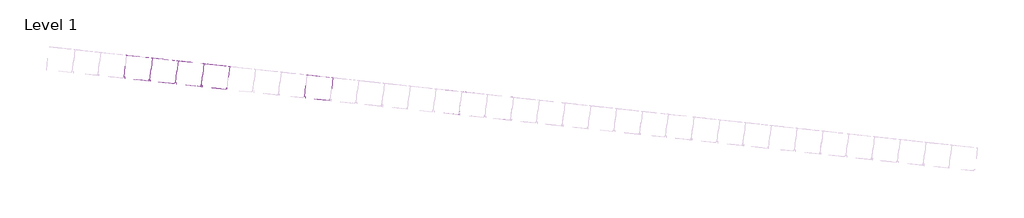
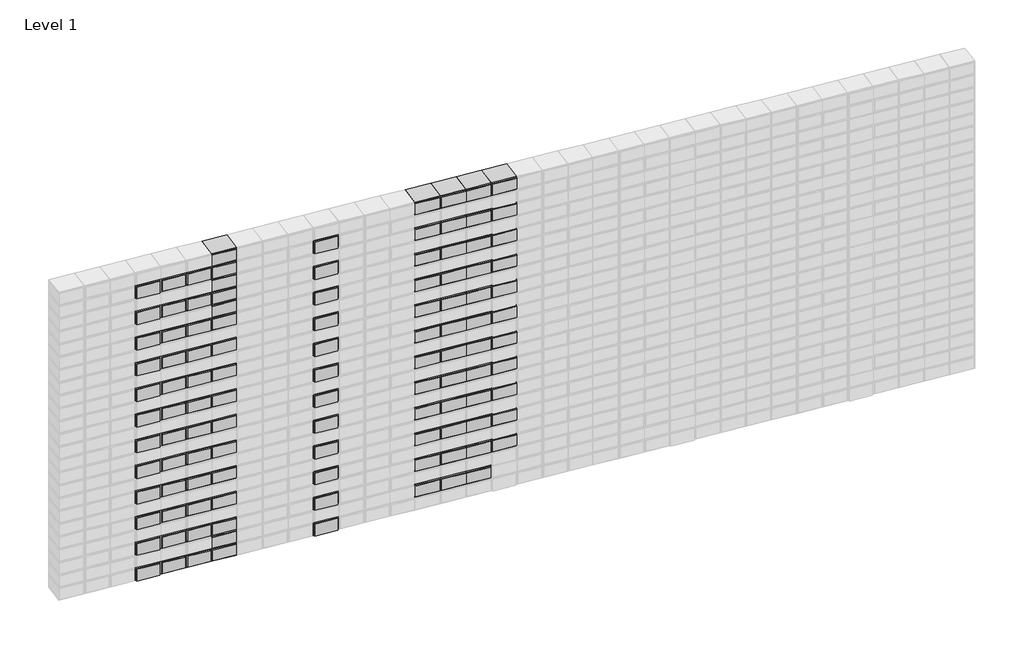
# One storey, part 13 of 18: 111 proxies.
"""IFC4 building model written with IfcOpenShell, lengths in millimetres."""

import ifcopenshell
import ifcopenshell.guid

model = None  # the IFC model being written
_history = None  # IfcOwnerHistory: only IFC2X3 demands one
_inside = {}  # id of a spatial element -> (the spatial element, [elements in it])
_under = {}  # id of a project, library or spatial element -> (it, [spatial elements below it])
_declared = {}  # id of a project -> (the project, [libraries it declares])
_typed = {}  # id of a type object -> (the type object, [elements of that type])
_made_of = {}  # id of a material, layer set ... -> (it, [elements and type objects made of it])


def new_model(schema):
    """Start an empty IFC model of exactly this schema.

    Asked for "IFC4X3", IfcOpenShell would pick the latest addendum, in which some entities
    have other attributes; the version numbers below select the first issue.
    IFC2X3 requires an IfcOwnerHistory on every rooted entity: one is made here for all.
    """
    global model, _history
    if schema == "IFC4X3":
        model = ifcopenshell.file(schema_version=(4, 3, 0, 0))
    else:
        model = ifcopenshell.file(schema=schema)
    _inside.clear()
    _under.clear()
    _declared.clear()
    _typed.clear()
    _made_of.clear()
    _history = None
    if model.schema == "IFC2X3":
        org = make("IfcOrganization", Name="unknown")
        user = make(
            "IfcPersonAndOrganization",
            ThePerson=make("IfcPerson", FamilyName="unknown"),
            TheOrganization=org,
        )
        app = make(
            "IfcApplication",
            ApplicationDeveloper=org,
            Version="unknown",
            ApplicationFullName="unknown",
            ApplicationIdentifier="unknown",
        )
        _history = make(
            "IfcOwnerHistory",
            OwningUser=user,
            OwningApplication=app,
            ChangeAction="ADDED",
            CreationDate=0,
        )
    return model


def make(cls, **values):
    """One entity of the class cls with the attributes given. An attribute that is None is left unset."""
    return model.create_entity(
        cls, **{name: value for name, value in values.items() if value is not None}
    )


def rooted(cls, **values):
    """An entity with a GlobalId (a new one), such as an element, a storey or a relation."""
    return make(cls, GlobalId=ifcopenshell.guid.new(), OwnerHistory=_history, **values)


def si_unit(unit_type, name, prefix=None):
    """IfcSIUnit, for example si_unit("LENGTHUNIT", "METRE", prefix="MILLI")."""
    return make("IfcSIUnit", UnitType=unit_type, Prefix=prefix, Name=name)


def assignment(units):
    """IfcUnitAssignment: the units of a project."""
    return None if units is None else make("IfcUnitAssignment", Units=units)


def point(xyz):
    """IfcCartesianPoint."""
    return None if xyz is None else make("IfcCartesianPoint", Coordinates=xyz)


def direction(xyz):
    """IfcDirection."""
    return None if xyz is None else make("IfcDirection", DirectionRatios=xyz)


def frame(location, z_axis=None, x_axis=None):
    """IfcAxis2Placement3D, a coordinate frame: its origin and axes. An axis left out is left unset."""
    return make(
        "IfcAxis2Placement3D",
        Location=point(location),
        Axis=direction(z_axis),
        RefDirection=direction(x_axis),
    )


def origin():
    """The frame at (0, 0, 0) with its axes left unset."""
    return frame((0.0, 0.0, 0.0))


def origin_with_axes():
    """The frame at (0, 0, 0) with the z axis (0, 0, 1) and the x axis (1, 0, 0) written out."""
    return frame((0.0, 0.0, 0.0), z_axis=(0.0, 0.0, 1.0), x_axis=(1.0, 0.0, 0.0))


def place(relative_to, where):
    """IfcLocalPlacement: puts the frame where relative to a parent placement (None: the world)."""
    return make(
        "IfcLocalPlacement", PlacementRelTo=relative_to, RelativePlacement=where
    )


def context(
    kind, dimensions, precision=None, world=None, true_north=None, identifier=None
):
    """IfcGeometricRepresentationContext, for example the 3D "Model" context."""
    return make(
        "IfcGeometricRepresentationContext",
        ContextIdentifier=identifier,
        ContextType=kind,
        CoordinateSpaceDimension=dimensions,
        Precision=precision,
        WorldCoordinateSystem=world,
        TrueNorth=true_north,
    )


def project(units=None, contexts=None):
    """IfcProject with its units and contexts."""
    return rooted(
        "IfcProject",
        Name="project",
        RepresentationContexts=contexts,
        UnitsInContext=assignment(units),
    )


def spatial(cls, under=None, at=None, **own):
    """A site, building, storey or space (cls), placed at a placement, below another one or the project."""
    s = rooted(cls, ObjectPlacement=at, **own)
    if under is not None:
        _under.setdefault(under.id(), (under, []))[1].append(s)
    return s


def polyline(points):
    """IfcPolyline through the points."""
    return make("IfcPolyline", Points=[point(p) for p in points])


def outline(outer, holes=None, kind="AREA"):
    """IfcArbitraryClosedProfileDef: a profile drawn as a closed curve; with holes, ...WithVoids."""
    if holes is None:
        return make("IfcArbitraryClosedProfileDef", ProfileType=kind, OuterCurve=outer)
    return make(
        "IfcArbitraryProfileDefWithVoids",
        ProfileType=kind,
        OuterCurve=outer,
        InnerCurves=holes,
    )


def extrude(swept, where, along, depth):
    """IfcExtrudedAreaSolid: the profile swept, set in the frame where, extruded along a direction by depth."""
    return make(
        "IfcExtrudedAreaSolid",
        SweptArea=swept,
        Position=where,
        ExtrudedDirection=direction(along),
        Depth=depth,
    )


def shape(context_of_items, identifier, shape_type, items):
    """IfcShapeRepresentation: the items that make up one representation, for example the "Body"."""
    return make(
        "IfcShapeRepresentation",
        ContextOfItems=context_of_items,
        RepresentationIdentifier=identifier,
        RepresentationType=shape_type,
        Items=items,
    )


def source(mapping_origin, context_of_items, identifier, shape_type, items):
    """IfcRepresentationMap: a shape defined once, which mapped items show again and again."""
    return make(
        "IfcRepresentationMap",
        MappingOrigin=mapping_origin,
        MappedRepresentation=shape(context_of_items, identifier, shape_type, items),
    )


def transform(
    local_origin,
    x_axis=None,
    y_axis=None,
    z_axis=None,
    scale=None,
    scale2=None,
    scale3=None,
    uniform=True,
):
    """IfcCartesianTransformationOperator3D, or its non-uniform kind. x_axis, y_axis, z_axis: its Axis1, 2, 3."""
    if uniform:
        return make(
            "IfcCartesianTransformationOperator3D",
            Axis1=direction(x_axis),
            Axis2=direction(y_axis),
            LocalOrigin=point(local_origin),
            Scale=scale,
            Axis3=direction(z_axis),
        )
    return make(
        "IfcCartesianTransformationOperator3DnonUniform",
        Axis1=direction(x_axis),
        Axis2=direction(y_axis),
        LocalOrigin=point(local_origin),
        Scale=scale,
        Axis3=direction(z_axis),
        Scale2=scale2,
        Scale3=scale3,
    )


def mapped(mapping_source, mapping_target):
    """IfcMappedItem: shows the shape of a source again, moved by a transform."""
    return make(
        "IfcMappedItem", MappingSource=mapping_source, MappingTarget=mapping_target
    )


def made_of(thing, what):
    """Note that an element or type object is made of a material, layer set ...; save() writes the relation."""
    if what is not None:
        _made_of.setdefault(what.id(), (what, []))[1].append(thing)
    return thing


def element(
    cls,
    number,
    at=None,
    inside=None,
    cuts=None,
    type_object=None,
    material=None,
    context=None,
    identifier="Body",
    shape_type=None,
    held_by="IfcProductDefinitionShape",
    body=None,
    shapes=None,
    **own,
):
    """One element of the class cls, such as IfcWall. Its Tag is "e" and its number.

    at: its placement. inside: the storey or other place that contains it. cuts: it is an
    opening in that element (IfcRelVoidsElement). A single representation is given by context,
    identifier, shape_type and body (its items); several are given by shapes. held_by: the class
    of the entity that holds the representations. save() writes the other relations.
    """
    e = rooted(cls, Tag="e%d" % number, ObjectPlacement=at, **own)
    if body is not None:
        shapes = [shape(context, identifier, shape_type, body)]
    if shapes is not None:
        e.Representation = make(held_by, Representations=shapes)
    if inside is not None:
        _inside.setdefault(inside.id(), (inside, []))[1].append(e)
    if cuts is not None:
        rooted(
            "IfcRelVoidsElement", RelatingBuildingElement=cuts, RelatedOpeningElement=e
        )
    if type_object is not None:
        _typed.setdefault(type_object.id(), (type_object, []))[1].append(e)
    return made_of(e, material)


def aggregate(whole, parts):
    """IfcRelAggregates: a whole, such as a stair, and the parts it consists of."""
    return rooted("IfcRelAggregates", RelatingObject=whole, RelatedObjects=parts)


def save(model, path):
    """Write the relations noted so far, then the file.

    IfcRelAggregates (storeys below a building ...), IfcRelContainedInSpatialStructure (elements
    in a storey), IfcRelDefinesByType, IfcRelAssociatesMaterial and IfcRelDeclares: one each for
    every whole, place, type object, material and project.
    """
    for whole, parts in _under.values():
        aggregate(whole, parts)
    for where, things in _inside.values():
        rooted(
            "IfcRelContainedInSpatialStructure",
            RelatedElements=things,
            RelatingStructure=where,
        )
    for kind, things in _typed.values():
        rooted("IfcRelDefinesByType", RelatedObjects=things, RelatingType=kind)
    for what, things in _made_of.values():
        rooted("IfcRelAssociatesMaterial", RelatedObjects=things, RelatingMaterial=what)
    for by, libraries in _declared.values():
        rooted("IfcRelDeclares", RelatingContext=by, RelatedDefinitions=libraries)
    model.write(path)


def geel_a5fc7152(model_context):
    return source(origin(), model_context, "Body", "SweptSolid", [
        extrude(outline(polyline([(131.1871262, 51.8695461), (24.8461542, 24.0369432), (23.5801491, 28.8740117), (125.0840527, 55.4406095), (111.9430518, 105.6488784), (10.4391482, 79.0822806), (9.1731432, 83.919349), (115.5141152, 111.7519519), (131.1871262, 51.8695461)])), origin_with_axes(), (0.0, 0.0, 1.0), 95.0),
        extrude(outline(polyline([(111.9430518, 105.6488784), (125.0840527, 55.4406095), (23.5801491, 28.8740117), (10.4391482, 79.0822806), (111.9430518, 105.6488784)])), origin_with_axes(), (0.0, 0.0, 1.0), 100.0),
    ])


def geel_ff5a4212(model_context):
    return source(origin(), model_context, "Body", "SweptSolid", [
        extrude(outline(polyline([(24.8461542, 24.0369432), (9.1731432, 83.919349), (115.5141152, 111.7519519), (116.7801202, 106.9148835), (15.2762167, 80.3482856), (28.4172176, 30.1400167), (129.9211211, 56.7066146), (131.1871262, 51.8695461), (24.8461542, 24.0369432)])), origin_with_axes(), (0.0, 0.0, 1.0), 95.0),
        extrude(outline(polyline([(116.7801202, 106.9148835), (129.9211211, 56.7066146), (28.4172176, 30.1400167), (15.2762167, 80.3482856), (116.7801202, 106.9148835)])), origin_with_axes(), (0.0, 0.0, 1.0), 100.0),
    ])


def rood_14a66368(model_context):
    return source(origin(), model_context, "Body", "SweptSolid", [
        extrude(outline(polyline([(24.8461542, 24.0369432), (9.1731432, 83.919349), (115.5141152, 111.7519519), (131.1871262, 51.8695461), (24.8461542, 24.0369432)]), holes=[polyline([(125.0840527, 55.4406095), (111.9430518, 105.6488784), (15.2762167, 80.3482856), (28.4172176, 30.1400167), (125.0840527, 55.4406095)])]), origin_with_axes(), (0.0, 0.0, 1.0), 95.0),
        extrude(outline(polyline([(111.9430518, 105.6488784), (125.0840527, 55.4406095), (28.4172176, 30.1400167), (15.2762167, 80.3482856), (111.9430518, 105.6488784)])), origin_with_axes(), (0.0, 0.0, 1.0), 100.0),
    ])


def rood_2ddd8018(model_context):
    return source(origin(), model_context, "Body", "SweptSolid", [
        extrude(outline(polyline([(24.8461542, 24.0369432), (9.1731432, 83.919349), (115.5141152, 111.7519519), (131.1871262, 51.8695461), (126.3500577, 50.6035411), (111.9430518, 105.6488784), (15.2762167, 80.3482856), (29.6832226, 25.3029482), (24.8461542, 24.0369432)])), origin_with_axes(), (0.0, 0.0, 1.0), 95.0),
        extrude(outline(polyline([(111.9430518, 105.6488784), (126.3500577, 50.6035411), (29.6832226, 25.3029482), (15.2762167, 80.3482856), (111.9430518, 105.6488784)])), origin_with_axes(), (0.0, 0.0, 1.0), 100.0),
    ])


model = new_model("IFC4")

# Units and contexts
model_context = context("Model", 3, world=origin())
ifc_project = project(units=[si_unit("LENGTHUNIT", "METRE", prefix="MILLI")], contexts=[model_context])

# Site, building, storey
site = spatial("IfcSite", under=ifc_project)
building = spatial("IfcBuilding", under=site)
storey = spatial("IfcBuildingStorey", under=building, Name="Level 1", Elevation=0.0)

# Proxies
placement = place(None, origin())
geel_shape = geel_a5fc7152(model_context)
element("IfcBuildingElementProxy", 1, Name="Geel", ObjectType="Geel", at=placement, inside=storey, context=model_context, shape_type="MappedRepresentation", body=[
    mapped(geel_shape, transform((10406.9656935, -4442.8724558, 2168.7358475), x_axis=(0.9617275503729374, -0.1047347566147725, -0.25320100633787673), y_axis=(0.25171277368869216, -0.02741220845642974, 0.9674136914420255), z_axis=(-0.10826263628609081, -0.9941223272738551, 0.0))),
])
element("IfcBuildingElementProxy", 2, Name="Geel", ObjectType="Geel", at=placement, inside=storey, context=model_context, shape_type="MappedRepresentation", body=[
    mapped(geel_shape, transform((10406.9656935, -4442.8724558, 2292.5348104), x_axis=(0.9617275503729374, -0.1047347566147725, -0.25320100633787673), y_axis=(0.25171277368869216, -0.02741220845642974, 0.9674136914420255), z_axis=(-0.10826263628609081, -0.9941223272738551, 0.0))),
])
element("IfcBuildingElementProxy", 3, Name="Geel", ObjectType="Geel", at=placement, inside=storey, context=model_context, shape_type="MappedRepresentation", body=[
    mapped(geel_shape, transform((10406.9656935, -4442.8724558, 2416.3337732), x_axis=(0.9617275503729384, -0.1047347566147726, -0.25320100633787307), y_axis=(0.25171277368868855, -0.02741220845642934, 0.9674136914420265), z_axis=(-0.10826263628609081, -0.994122327273855, 0.0))),
])
element("IfcBuildingElementProxy", 4, Name="Geel", ObjectType="Geel", at=placement, inside=storey, context=model_context, shape_type="MappedRepresentation", body=[
    mapped(geel_shape, transform((10406.9656935, -4442.8724558, 2540.132736), x_axis=(0.9617275503729374, -0.1047347566147725, -0.25320100633787673), y_axis=(0.25171277368869216, -0.02741220845642974, 0.9674136914420255), z_axis=(-0.10826263628609081, -0.9941223272738551, 0.0))),
])
element("IfcBuildingElementProxy", 5, Name="Geel", ObjectType="Geel", at=placement, inside=storey, context=model_context, shape_type="MappedRepresentation", body=[
    mapped(geel_shape, transform((10406.9656935, -4442.8724558, 2663.9316989), x_axis=(0.9617275503729374, -0.1047347566147725, -0.25320100633787673), y_axis=(0.25171277368869216, -0.02741220845642974, 0.9674136914420255), z_axis=(-0.10826263628609081, -0.9941223272738551, 0.0))),
])
element("IfcBuildingElementProxy", 6, Name="Geel", ObjectType="Geel", at=placement, inside=storey, context=model_context, shape_type="MappedRepresentation", body=[
    mapped(geel_shape, transform((10406.9656935, -4442.8724558, 2787.7306617), x_axis=(0.9617275503729374, -0.1047347566147725, -0.25320100633787673), y_axis=(0.25171277368869216, -0.02741220845642974, 0.9674136914420255), z_axis=(-0.10826263628609081, -0.9941223272738551, 0.0))),
])
element("IfcBuildingElementProxy", 7, Name="Geel", ObjectType="Geel", at=placement, inside=storey, context=model_context, shape_type="MappedRepresentation", body=[
    mapped(geel_shape, transform((10406.9656935, -4442.8724558, 2911.5296245), x_axis=(0.9617275503729374, -0.1047347566147725, -0.25320100633787673), y_axis=(0.25171277368869216, -0.02741220845642974, 0.9674136914420255), z_axis=(-0.10826263628609081, -0.9941223272738551, 0.0))),
])
element("IfcBuildingElementProxy", 8, Name="Geel", ObjectType="Geel", at=placement, inside=storey, context=model_context, shape_type="MappedRepresentation", body=[
    mapped(geel_shape, transform((10406.9656935, -4442.8724558, 3035.3285874), x_axis=(0.9617275503729374, -0.1047347566147725, -0.25320100633787673), y_axis=(0.25171277368869216, -0.02741220845642974, 0.9674136914420255), z_axis=(-0.10826263628609081, -0.9941223272738551, 0.0))),
])
element("IfcBuildingElementProxy", 9, Name="Geel", ObjectType="Geel", at=placement, inside=storey, context=model_context, shape_type="MappedRepresentation", body=[
    mapped(geel_shape, transform((10406.9656935, -4442.8724558, 3159.1275502), x_axis=(0.9617275503729374, -0.1047347566147725, -0.25320100633787673), y_axis=(0.25171277368869216, -0.02741220845642974, 0.9674136914420255), z_axis=(-0.10826263628609081, -0.9941223272738551, 0.0))),
])
element("IfcBuildingElementProxy", 10, Name="Geel", ObjectType="Geel", at=placement, inside=storey, context=model_context, shape_type="MappedRepresentation", body=[
    mapped(geel_shape, transform((10406.9656935, -4442.8724558, 3282.926513), x_axis=(0.9617275503729374, -0.1047347566147725, -0.25320100633787673), y_axis=(0.25171277368869216, -0.02741220845642974, 0.9674136914420255), z_axis=(-0.10826263628609081, -0.9941223272738551, 0.0))),
])
element("IfcBuildingElementProxy", 11, Name="Geel", ObjectType="Geel", at=placement, inside=storey, context=model_context, shape_type="MappedRepresentation", body=[
    mapped(geel_shape, transform((10406.9656935, -4442.8724558, 3406.7254759), x_axis=(0.9617275503729374, -0.1047347566147725, -0.25320100633787673), y_axis=(0.25171277368869216, -0.02741220845642974, 0.9674136914420255), z_axis=(-0.10826263628609081, -0.9941223272738551, 0.0))),
])
element("IfcBuildingElementProxy", 12, Name="Geel", ObjectType="Geel", at=placement, inside=storey, context=model_context, shape_type="MappedRepresentation", body=[
    mapped(geel_shape, transform((10406.9656935, -4442.8724558, 2044.9368847), x_axis=(0.9617275503729384, -0.1047347566147726, -0.25320100633787307), y_axis=(0.25171277368868855, -0.02741220845642934, 0.9674136914420265), z_axis=(-0.10826263628609081, -0.994122327273855, 0.0))),
])
element("IfcBuildingElementProxy", 13, Name="Geel", ObjectType="Geel", at=placement, inside=storey, context=model_context, shape_type="MappedRepresentation", body=[
    mapped(geel_shape, transform((10625.5194219, -4466.6735537, 2168.7358475), x_axis=(0.9617275503729374, -0.1047347566147725, -0.25320100633787673), y_axis=(0.25171277368869216, -0.02741220845642974, 0.9674136914420255), z_axis=(-0.10826263628609081, -0.9941223272738551, 0.0))),
])
element("IfcBuildingElementProxy", 14, Name="Geel", ObjectType="Geel", at=placement, inside=storey, context=model_context, shape_type="MappedRepresentation", body=[
    mapped(geel_shape, transform((10625.5194219, -4466.6735537, 2292.5348104), x_axis=(0.9617275503729374, -0.1047347566147725, -0.25320100633787673), y_axis=(0.25171277368869216, -0.02741220845642974, 0.9674136914420255), z_axis=(-0.10826263628609081, -0.9941223272738551, 0.0))),
])
element("IfcBuildingElementProxy", 15, Name="Geel", ObjectType="Geel", at=placement, inside=storey, context=model_context, shape_type="MappedRepresentation", body=[
    mapped(geel_shape, transform((10625.5194219, -4466.6735537, 2416.3337732), x_axis=(0.9617275503729384, -0.1047347566147726, -0.25320100633787307), y_axis=(0.25171277368868855, -0.02741220845642934, 0.9674136914420265), z_axis=(-0.10826263628609081, -0.994122327273855, 0.0))),
])
element("IfcBuildingElementProxy", 16, Name="Geel", ObjectType="Geel", at=placement, inside=storey, context=model_context, shape_type="MappedRepresentation", body=[
    mapped(geel_shape, transform((10625.5194219, -4466.6735537, 2540.132736), x_axis=(0.9617275503729374, -0.1047347566147725, -0.25320100633787673), y_axis=(0.25171277368869216, -0.02741220845642974, 0.9674136914420255), z_axis=(-0.10826263628609081, -0.9941223272738551, 0.0))),
])
element("IfcBuildingElementProxy", 17, Name="Geel", ObjectType="Geel", at=placement, inside=storey, context=model_context, shape_type="MappedRepresentation", body=[
    mapped(geel_shape, transform((10625.5194219, -4466.6735537, 2663.9316989), x_axis=(0.9617275503729374, -0.1047347566147725, -0.25320100633787673), y_axis=(0.25171277368869216, -0.02741220845642974, 0.9674136914420255), z_axis=(-0.10826263628609081, -0.9941223272738551, 0.0))),
])
element("IfcBuildingElementProxy", 18, Name="Geel", ObjectType="Geel", at=placement, inside=storey, context=model_context, shape_type="MappedRepresentation", body=[
    mapped(geel_shape, transform((10625.5194219, -4466.6735537, 2787.7306617), x_axis=(0.9617275503729374, -0.1047347566147725, -0.25320100633787673), y_axis=(0.25171277368869216, -0.02741220845642974, 0.9674136914420255), z_axis=(-0.10826263628609081, -0.9941223272738551, 0.0))),
])
element("IfcBuildingElementProxy", 19, Name="Geel", ObjectType="Geel", at=placement, inside=storey, context=model_context, shape_type="MappedRepresentation", body=[
    mapped(geel_shape, transform((10625.5194219, -4466.6735537, 2911.5296245), x_axis=(0.9617275503729374, -0.1047347566147725, -0.25320100633787673), y_axis=(0.25171277368869216, -0.02741220845642974, 0.9674136914420255), z_axis=(-0.10826263628609081, -0.9941223272738551, 0.0))),
])
element("IfcBuildingElementProxy", 20, Name="Geel", ObjectType="Geel", at=placement, inside=storey, context=model_context, shape_type="MappedRepresentation", body=[
    mapped(geel_shape, transform((10625.5194219, -4466.6735537, 3035.3285874), x_axis=(0.9617275503729374, -0.1047347566147725, -0.25320100633787673), y_axis=(0.25171277368869216, -0.02741220845642974, 0.9674136914420255), z_axis=(-0.10826263628609081, -0.9941223272738551, 0.0))),
])
element("IfcBuildingElementProxy", 21, Name="Geel", ObjectType="Geel", at=placement, inside=storey, context=model_context, shape_type="MappedRepresentation", body=[
    mapped(geel_shape, transform((10625.5194219, -4466.6735537, 3159.1275502), x_axis=(0.9617275503729374, -0.1047347566147725, -0.25320100633787673), y_axis=(0.25171277368869216, -0.02741220845642974, 0.9674136914420255), z_axis=(-0.10826263628609081, -0.9941223272738551, 0.0))),
])
element("IfcBuildingElementProxy", 22, Name="Geel", ObjectType="Geel", at=placement, inside=storey, context=model_context, shape_type="MappedRepresentation", body=[
    mapped(geel_shape, transform((10625.5194219, -4466.6735537, 3282.926513), x_axis=(0.9617275503729374, -0.1047347566147725, -0.25320100633787673), y_axis=(0.25171277368869216, -0.02741220845642974, 0.9674136914420255), z_axis=(-0.10826263628609081, -0.9941223272738551, 0.0))),
])
element("IfcBuildingElementProxy", 23, Name="Geel", ObjectType="Geel", at=placement, inside=storey, context=model_context, shape_type="MappedRepresentation", body=[
    mapped(geel_shape, transform((10625.5194219, -4466.6735537, 3406.7254759), x_axis=(0.9617275503729374, -0.1047347566147725, -0.25320100633787673), y_axis=(0.25171277368869216, -0.02741220845642974, 0.9674136914420255), z_axis=(-0.10826263628609081, -0.9941223272738551, 0.0))),
])
element("IfcBuildingElementProxy", 24, Name="Geel", ObjectType="Geel", at=placement, inside=storey, context=model_context, shape_type="MappedRepresentation", body=[
    mapped(geel_shape, transform((10625.5194219, -4466.6735537, 2044.9368847), x_axis=(0.9617275503729384, -0.1047347566147726, -0.25320100633787307), y_axis=(0.25171277368868855, -0.02741220845642934, 0.9674136914420265), z_axis=(-0.10826263628609081, -0.994122327273855, 0.0))),
])
element("IfcBuildingElementProxy", 25, Name="Geel", ObjectType="Geel", at=placement, inside=storey, context=model_context, shape_type="MappedRepresentation", body=[
    mapped(geel_shape, transform((9532.7507801, -4347.6680644, 3159.1275502), x_axis=(0.9617275503729374, -0.1047347566147725, -0.25320100633787673), y_axis=(0.25171277368869216, -0.02741220845642974, 0.9674136914420255), z_axis=(-0.10826263628609081, -0.9941223272738551, 0.0))),
])
element("IfcBuildingElementProxy", 26, Name="Geel", ObjectType="Geel", at=placement, inside=storey, context=model_context, shape_type="MappedRepresentation", body=[
    mapped(geel_shape, transform((9532.7507801, -4347.6680644, 3282.926513), x_axis=(0.9617275503729374, -0.1047347566147725, -0.25320100633787673), y_axis=(0.25171277368869216, -0.02741220845642974, 0.9674136914420255), z_axis=(-0.10826263628609081, -0.9941223272738551, 0.0))),
])
element("IfcBuildingElementProxy", 27, Name="Geel", ObjectType="Geel", at=placement, inside=storey, context=model_context, shape_type="MappedRepresentation", body=[
    mapped(geel_shape, transform((9532.7507801, -4347.6680644, 3406.7254759), x_axis=(0.9617275503729374, -0.1047347566147725, -0.25320100633787673), y_axis=(0.25171277368869216, -0.02741220845642974, 0.9674136914420255), z_axis=(-0.10826263628609081, -0.9941223272738551, 0.0))),
])
element("IfcBuildingElementProxy", 28, Name="Geel", ObjectType="Geel", at=placement, inside=storey, context=model_context, shape_type="MappedRepresentation", body=[
    mapped(geel_shape, transform((9532.7507801, -4347.6680644, 2044.9368847), x_axis=(0.9617275503729384, -0.1047347566147726, -0.25320100633787307), y_axis=(0.25171277368868855, -0.02741220845642934, 0.9674136914420265), z_axis=(-0.10826263628609081, -0.994122327273855, 0.0))),
])
geel_2_shape = geel_ff5a4212(model_context)
element("IfcBuildingElementProxy", 29, Name="Geel", ObjectType="Geel", at=placement, inside=storey, context=model_context, shape_type="MappedRepresentation", body=[
    mapped(geel_2_shape, transform((10516.2425577, -4454.7730048, 2168.7358475), x_axis=(0.9617275503729374, -0.1047347566147725, -0.25320100633787673), y_axis=(0.25171277368869216, -0.02741220845642974, 0.9674136914420255), z_axis=(-0.10826263628609081, -0.9941223272738551, 0.0))),
])
element("IfcBuildingElementProxy", 30, Name="Geel", ObjectType="Geel", at=placement, inside=storey, context=model_context, shape_type="MappedRepresentation", body=[
    mapped(geel_2_shape, transform((10516.2425577, -4454.7730048, 2292.5348104), x_axis=(0.9617275503729374, -0.1047347566147725, -0.25320100633787673), y_axis=(0.25171277368869216, -0.02741220845642974, 0.9674136914420255), z_axis=(-0.10826263628609081, -0.9941223272738551, 0.0))),
])
element("IfcBuildingElementProxy", 31, Name="Geel", ObjectType="Geel", at=placement, inside=storey, context=model_context, shape_type="MappedRepresentation", body=[
    mapped(geel_2_shape, transform((10516.2425577, -4454.7730048, 2416.3337732), x_axis=(0.9617275503729384, -0.1047347566147726, -0.25320100633787307), y_axis=(0.25171277368868855, -0.02741220845642934, 0.9674136914420265), z_axis=(-0.10826263628609081, -0.994122327273855, 0.0))),
])
element("IfcBuildingElementProxy", 32, Name="Geel", ObjectType="Geel", at=placement, inside=storey, context=model_context, shape_type="MappedRepresentation", body=[
    mapped(geel_2_shape, transform((10516.2425577, -4454.7730048, 2540.132736), x_axis=(0.9617275503729374, -0.1047347566147725, -0.25320100633787673), y_axis=(0.25171277368869216, -0.02741220845642974, 0.9674136914420255), z_axis=(-0.10826263628609081, -0.9941223272738551, 0.0))),
])
element("IfcBuildingElementProxy", 33, Name="Geel", ObjectType="Geel", at=placement, inside=storey, context=model_context, shape_type="MappedRepresentation", body=[
    mapped(geel_2_shape, transform((10516.2425577, -4454.7730048, 2663.9316989), x_axis=(0.9617275503729374, -0.1047347566147725, -0.25320100633787673), y_axis=(0.25171277368869216, -0.02741220845642974, 0.9674136914420255), z_axis=(-0.10826263628609081, -0.9941223272738551, 0.0))),
])
element("IfcBuildingElementProxy", 34, Name="Geel", ObjectType="Geel", at=placement, inside=storey, context=model_context, shape_type="MappedRepresentation", body=[
    mapped(geel_2_shape, transform((10516.2425577, -4454.7730048, 2787.7306617), x_axis=(0.9617275503729374, -0.1047347566147725, -0.25320100633787673), y_axis=(0.25171277368869216, -0.02741220845642974, 0.9674136914420255), z_axis=(-0.10826263628609081, -0.9941223272738551, 0.0))),
])
element("IfcBuildingElementProxy", 35, Name="Geel", ObjectType="Geel", at=placement, inside=storey, context=model_context, shape_type="MappedRepresentation", body=[
    mapped(geel_2_shape, transform((10516.2425577, -4454.7730048, 2911.5296245), x_axis=(0.9617275503729374, -0.1047347566147725, -0.25320100633787673), y_axis=(0.25171277368869216, -0.02741220845642974, 0.9674136914420255), z_axis=(-0.10826263628609081, -0.9941223272738551, 0.0))),
])
element("IfcBuildingElementProxy", 36, Name="Geel", ObjectType="Geel", at=placement, inside=storey, context=model_context, shape_type="MappedRepresentation", body=[
    mapped(geel_2_shape, transform((10516.2425577, -4454.7730048, 3035.3285874), x_axis=(0.9617275503729374, -0.1047347566147725, -0.25320100633787673), y_axis=(0.25171277368869216, -0.02741220845642974, 0.9674136914420255), z_axis=(-0.10826263628609081, -0.9941223272738551, 0.0))),
])
element("IfcBuildingElementProxy", 37, Name="Geel", ObjectType="Geel", at=placement, inside=storey, context=model_context, shape_type="MappedRepresentation", body=[
    mapped(geel_2_shape, transform((10516.2425577, -4454.7730048, 3159.1275502), x_axis=(0.9617275503729374, -0.1047347566147725, -0.25320100633787673), y_axis=(0.25171277368869216, -0.02741220845642974, 0.9674136914420255), z_axis=(-0.10826263628609081, -0.9941223272738551, 0.0))),
])
element("IfcBuildingElementProxy", 38, Name="Geel", ObjectType="Geel", at=placement, inside=storey, context=model_context, shape_type="MappedRepresentation", body=[
    mapped(geel_2_shape, transform((10516.2425577, -4454.7730048, 3282.926513), x_axis=(0.9617275503729374, -0.1047347566147725, -0.25320100633787673), y_axis=(0.25171277368869216, -0.02741220845642974, 0.9674136914420255), z_axis=(-0.10826263628609081, -0.9941223272738551, 0.0))),
])
element("IfcBuildingElementProxy", 39, Name="Geel", ObjectType="Geel", at=placement, inside=storey, context=model_context, shape_type="MappedRepresentation", body=[
    mapped(geel_2_shape, transform((10516.2425577, -4454.7730048, 3406.7254759), x_axis=(0.9617275503729374, -0.1047347566147725, -0.25320100633787673), y_axis=(0.25171277368869216, -0.02741220845642974, 0.9674136914420255), z_axis=(-0.10826263628609081, -0.9941223272738551, 0.0))),
])
element("IfcBuildingElementProxy", 40, Name="Geel", ObjectType="Geel", at=placement, inside=storey, context=model_context, shape_type="MappedRepresentation", body=[
    mapped(geel_2_shape, transform((10516.2425577, -4454.7730048, 2044.9368847), x_axis=(0.9617275503729384, -0.1047347566147726, -0.25320100633787307), y_axis=(0.25171277368868855, -0.02741220845642934, 0.9674136914420265), z_axis=(-0.10826263628609081, -0.994122327273855, 0.0))),
])
element("IfcBuildingElementProxy", 41, Name="Geel", ObjectType="Geel", at=placement, inside=storey, context=model_context, shape_type="MappedRepresentation", body=[
    mapped(geel_2_shape, transform((10734.7962861, -4478.5741026, 2168.7358475), x_axis=(0.961727550372942, -0.10473475661477027, -0.25320100633786047), y_axis=(0.2517127736886762, -0.02741220845642728, 0.9674136914420297), z_axis=(-0.10826263628608807, -0.9941223272738554, 0.0))),
])
element("IfcBuildingElementProxy", 42, Name="Geel", ObjectType="Geel", at=placement, inside=storey, context=model_context, shape_type="MappedRepresentation", body=[
    mapped(geel_2_shape, transform((10734.7962861, -4478.5741026, 2292.5348104), x_axis=(0.961727550372942, -0.10473475661477027, -0.25320100633786047), y_axis=(0.2517127736886762, -0.02741220845642728, 0.9674136914420297), z_axis=(-0.10826263628608807, -0.9941223272738554, 0.0))),
])
element("IfcBuildingElementProxy", 43, Name="Geel", ObjectType="Geel", at=placement, inside=storey, context=model_context, shape_type="MappedRepresentation", body=[
    mapped(geel_2_shape, transform((10734.7962861, -4478.5741026, 2416.3337732), x_axis=(0.961727550372943, -0.10473475661477039, -0.25320100633785686), y_axis=(0.25171277368867245, -0.02741220845642689, 0.9674136914420308), z_axis=(-0.10826263628608805, -0.9941223272738553, 0.0))),
])
element("IfcBuildingElementProxy", 44, Name="Geel", ObjectType="Geel", at=placement, inside=storey, context=model_context, shape_type="MappedRepresentation", body=[
    mapped(geel_2_shape, transform((10734.7962861, -4478.5741026, 2540.132736), x_axis=(0.961727550372942, -0.10473475661477027, -0.25320100633786047), y_axis=(0.2517127736886762, -0.02741220845642728, 0.9674136914420297), z_axis=(-0.10826263628608807, -0.9941223272738554, 0.0))),
])
element("IfcBuildingElementProxy", 45, Name="Geel", ObjectType="Geel", at=placement, inside=storey, context=model_context, shape_type="MappedRepresentation", body=[
    mapped(geel_2_shape, transform((10734.7962861, -4478.5741026, 2663.9316989), x_axis=(0.961727550372942, -0.10473475661477027, -0.25320100633786047), y_axis=(0.2517127736886762, -0.02741220845642728, 0.9674136914420297), z_axis=(-0.10826263628608807, -0.9941223272738554, 0.0))),
])
element("IfcBuildingElementProxy", 46, Name="Geel", ObjectType="Geel", at=placement, inside=storey, context=model_context, shape_type="MappedRepresentation", body=[
    mapped(geel_2_shape, transform((10734.7962861, -4478.5741026, 2787.7306617), x_axis=(0.961727550372942, -0.10473475661477027, -0.25320100633786047), y_axis=(0.2517127736886762, -0.02741220845642728, 0.9674136914420297), z_axis=(-0.10826263628608807, -0.9941223272738554, 0.0))),
])
element("IfcBuildingElementProxy", 47, Name="Geel", ObjectType="Geel", at=placement, inside=storey, context=model_context, shape_type="MappedRepresentation", body=[
    mapped(geel_2_shape, transform((10734.7962861, -4478.5741026, 2911.5296245), x_axis=(0.961727550372942, -0.10473475661477027, -0.25320100633786047), y_axis=(0.2517127736886762, -0.02741220845642728, 0.9674136914420297), z_axis=(-0.10826263628608807, -0.9941223272738554, 0.0))),
])
element("IfcBuildingElementProxy", 48, Name="Geel", ObjectType="Geel", at=placement, inside=storey, context=model_context, shape_type="MappedRepresentation", body=[
    mapped(geel_2_shape, transform((10734.7962861, -4478.5741026, 3035.3285874), x_axis=(0.961727550372942, -0.10473475661477027, -0.25320100633786047), y_axis=(0.2517127736886762, -0.02741220845642728, 0.9674136914420297), z_axis=(-0.10826263628608807, -0.9941223272738554, 0.0))),
])
element("IfcBuildingElementProxy", 49, Name="Geel", ObjectType="Geel", at=placement, inside=storey, context=model_context, shape_type="MappedRepresentation", body=[
    mapped(geel_2_shape, transform((10734.7962861, -4478.5741026, 3159.1275502), x_axis=(0.961727550372942, -0.10473475661477027, -0.25320100633786047), y_axis=(0.2517127736886762, -0.02741220845642728, 0.9674136914420297), z_axis=(-0.10826263628608807, -0.9941223272738554, 0.0))),
])
element("IfcBuildingElementProxy", 50, Name="Geel", ObjectType="Geel", at=placement, inside=storey, context=model_context, shape_type="MappedRepresentation", body=[
    mapped(geel_2_shape, transform((10734.7962861, -4478.5741026, 3282.926513), x_axis=(0.961727550372942, -0.10473475661477027, -0.25320100633786047), y_axis=(0.2517127736886762, -0.02741220845642728, 0.9674136914420297), z_axis=(-0.10826263628608807, -0.9941223272738554, 0.0))),
])
element("IfcBuildingElementProxy", 51, Name="Geel", ObjectType="Geel", at=placement, inside=storey, context=model_context, shape_type="MappedRepresentation", body=[
    mapped(geel_2_shape, transform((10734.7962861, -4478.5741026, 3406.7254759), x_axis=(0.961727550372942, -0.10473475661477027, -0.25320100633786047), y_axis=(0.2517127736886762, -0.02741220845642728, 0.9674136914420297), z_axis=(-0.10826263628608807, -0.9941223272738554, 0.0))),
])
rood_shape = rood_14a66368(model_context)
element("IfcBuildingElementProxy", 52, Name="Rood", ObjectType="Rood", at=placement, inside=storey, context=model_context, shape_type="MappedRepresentation", body=[
    mapped(rood_shape, transform((9314.1970517, -4323.8669665, 2106.8363661), x_axis=(0.9617275503729396, -0.10473475661477374, -0.25320100633786874), y_axis=(0.251712773688684, -0.027412208456429103, 0.9674136914420278), z_axis=(-0.10826263628609185, -0.994122327273855, 0.0))),
])
element("IfcBuildingElementProxy", 53, Name="Rood", ObjectType="Rood", at=placement, inside=storey, context=model_context, shape_type="MappedRepresentation", body=[
    mapped(rood_shape, transform((9314.1970517, -4323.8669665, 2230.6353289), x_axis=(0.9617275503729403, -0.10473475661477383, -0.253201006337865), y_axis=(0.2517127736886804, -0.0274122084564287, 0.9674136914420286), z_axis=(-0.10826263628609184, -0.9941223272738549, 0.0))),
])
element("IfcBuildingElementProxy", 54, Name="Rood", ObjectType="Rood", at=placement, inside=storey, context=model_context, shape_type="MappedRepresentation", body=[
    mapped(rood_shape, transform((9314.1970517, -4323.8669665, 2354.4342918), x_axis=(0.9617275503729396, -0.10473475661477374, -0.25320100633786874), y_axis=(0.251712773688684, -0.027412208456429103, 0.9674136914420278), z_axis=(-0.10826263628609185, -0.994122327273855, 0.0))),
])
element("IfcBuildingElementProxy", 55, Name="Rood", ObjectType="Rood", at=placement, inside=storey, context=model_context, shape_type="MappedRepresentation", body=[
    mapped(rood_shape, transform((9314.1970517, -4323.8669665, 2478.2332546), x_axis=(0.9617275503729396, -0.10473475661477374, -0.25320100633786874), y_axis=(0.251712773688684, -0.027412208456429103, 0.9674136914420278), z_axis=(-0.10826263628609185, -0.994122327273855, 0.0))),
])
element("IfcBuildingElementProxy", 56, Name="Rood", ObjectType="Rood", at=placement, inside=storey, context=model_context, shape_type="MappedRepresentation", body=[
    mapped(rood_shape, transform((9314.1970517, -4323.8669665, 2602.0322174), x_axis=(0.9617275503729414, -0.10473475661477394, -0.2532010063378615), y_axis=(0.25171277368867684, -0.027412208456428312, 0.9674136914420295), z_axis=(-0.10826263628609185, -0.9941223272738549, 0.0))),
])
element("IfcBuildingElementProxy", 57, Name="Rood", ObjectType="Rood", at=placement, inside=storey, context=model_context, shape_type="MappedRepresentation", body=[
    mapped(rood_shape, transform((9314.1970517, -4323.8669665, 2725.8311803), x_axis=(0.9617275503729396, -0.10473475661477374, -0.25320100633786874), y_axis=(0.251712773688684, -0.027412208456429103, 0.9674136914420278), z_axis=(-0.10826263628609185, -0.994122327273855, 0.0))),
])
element("IfcBuildingElementProxy", 58, Name="Rood", ObjectType="Rood", at=placement, inside=storey, context=model_context, shape_type="MappedRepresentation", body=[
    mapped(rood_shape, transform((9314.1970517, -4323.8669665, 2849.6301431), x_axis=(0.9617275503729396, -0.10473475661477374, -0.25320100633786874), y_axis=(0.251712773688684, -0.027412208456429103, 0.9674136914420278), z_axis=(-0.10826263628609185, -0.994122327273855, 0.0))),
])
element("IfcBuildingElementProxy", 59, Name="Rood", ObjectType="Rood", at=placement, inside=storey, context=model_context, shape_type="MappedRepresentation", body=[
    mapped(rood_shape, transform((9314.1970517, -4323.8669665, 2973.4291059), x_axis=(0.9617275503729396, -0.10473475661477374, -0.25320100633786874), y_axis=(0.251712773688684, -0.027412208456429103, 0.9674136914420278), z_axis=(-0.10826263628609185, -0.994122327273855, 0.0))),
])
element("IfcBuildingElementProxy", 60, Name="Rood", ObjectType="Rood", at=placement, inside=storey, context=model_context, shape_type="MappedRepresentation", body=[
    mapped(rood_shape, transform((9314.1970517, -4323.8669665, 3097.2280688), x_axis=(0.9617275503729414, -0.10473475661477394, -0.2532010063378615), y_axis=(0.25171277368867684, -0.027412208456428312, 0.9674136914420295), z_axis=(-0.10826263628609185, -0.9941223272738549, 0.0))),
])
element("IfcBuildingElementProxy", 61, Name="Rood", ObjectType="Rood", at=placement, inside=storey, context=model_context, shape_type="MappedRepresentation", body=[
    mapped(rood_shape, transform((9314.1970517, -4323.8669665, 3221.0270316), x_axis=(0.9617275503729396, -0.10473475661477374, -0.25320100633786874), y_axis=(0.251712773688684, -0.027412208456429103, 0.9674136914420278), z_axis=(-0.10826263628609185, -0.994122327273855, 0.0))),
])
element("IfcBuildingElementProxy", 62, Name="Rood", ObjectType="Rood", at=placement, inside=storey, context=model_context, shape_type="MappedRepresentation", body=[
    mapped(rood_shape, transform((9314.1970517, -4323.8669665, 3344.8259944), x_axis=(0.9617275503729377, -0.10473475661477352, -0.2532010063378758), y_axis=(0.2517127736886912, -0.027412208456429887, 0.9674136914420259), z_axis=(-0.10826263628609185, -0.9941223272738549, 0.0))),
])
element("IfcBuildingElementProxy", 63, Name="Rood", ObjectType="Rood", at=placement, inside=storey, context=model_context, shape_type="MappedRepresentation", body=[
    mapped(rood_shape, transform((9314.1970517, -4323.8669665, 1983.0374033), x_axis=(0.9617275503729396, -0.10473475661477374, -0.25320100633786874), y_axis=(0.251712773688684, -0.027412208456429103, 0.9674136914420278), z_axis=(-0.10826263628609185, -0.994122327273855, 0.0))),
])
element("IfcBuildingElementProxy", 64, Name="Rood", ObjectType="Rood", at=placement, inside=storey, context=model_context, shape_type="MappedRepresentation", body=[
    mapped(rood_shape, transform((9423.4739159, -4335.7675154, 2106.8363661), x_axis=(0.9617275503729402, -0.10473475661476898, -0.2532010063378681), y_axis=(0.25171277368868383, -0.02741220845642784, 0.9674136914420278), z_axis=(-0.10826263628608696, -0.9941223272738555, 0.0))),
])
element("IfcBuildingElementProxy", 65, Name="Rood", ObjectType="Rood", at=placement, inside=storey, context=model_context, shape_type="MappedRepresentation", body=[
    mapped(rood_shape, transform((9423.4739159, -4335.7675154, 2230.6353289), x_axis=(0.9617275503729411, -0.10473475661476908, -0.2532010063378646), y_axis=(0.25171277368868017, -0.027412208456427424, 0.9674136914420287), z_axis=(-0.10826263628608693, -0.9941223272738554, 0.0))),
])
element("IfcBuildingElementProxy", 66, Name="Rood", ObjectType="Rood", at=placement, inside=storey, context=model_context, shape_type="MappedRepresentation", body=[
    mapped(rood_shape, transform((9423.4739159, -4335.7675154, 2354.4342918), x_axis=(0.9617275503729402, -0.10473475661476898, -0.2532010063378681), y_axis=(0.25171277368868383, -0.02741220845642784, 0.9674136914420278), z_axis=(-0.10826263628608696, -0.9941223272738555, 0.0))),
])
element("IfcBuildingElementProxy", 67, Name="Rood", ObjectType="Rood", at=placement, inside=storey, context=model_context, shape_type="MappedRepresentation", body=[
    mapped(rood_shape, transform((9423.4739159, -4335.7675154, 2478.2332546), x_axis=(0.9617275503729402, -0.10473475661476898, -0.2532010063378681), y_axis=(0.25171277368868383, -0.02741220845642784, 0.9674136914420278), z_axis=(-0.10826263628608696, -0.9941223272738555, 0.0))),
])
element("IfcBuildingElementProxy", 68, Name="Rood", ObjectType="Rood", at=placement, inside=storey, context=model_context, shape_type="MappedRepresentation", body=[
    mapped(rood_shape, transform((9423.4739159, -4335.7675154, 2602.0322174), x_axis=(0.9617275503729421, -0.10473475661476919, -0.25320100633786086), y_axis=(0.25171277368867656, -0.02741220845642703, 0.9674136914420297), z_axis=(-0.10826263628608694, -0.9941223272738555, 0.0))),
])
element("IfcBuildingElementProxy", 69, Name="Rood", ObjectType="Rood", at=placement, inside=storey, context=model_context, shape_type="MappedRepresentation", body=[
    mapped(rood_shape, transform((9423.4739159, -4335.7675154, 2725.8311803), x_axis=(0.9617275503729402, -0.10473475661476898, -0.2532010063378681), y_axis=(0.25171277368868383, -0.02741220845642784, 0.9674136914420278), z_axis=(-0.10826263628608696, -0.9941223272738555, 0.0))),
])
element("IfcBuildingElementProxy", 70, Name="Rood", ObjectType="Rood", at=placement, inside=storey, context=model_context, shape_type="MappedRepresentation", body=[
    mapped(rood_shape, transform((9423.4739159, -4335.7675154, 2849.6301431), x_axis=(0.9617275503729402, -0.10473475661476898, -0.2532010063378681), y_axis=(0.25171277368868383, -0.02741220845642784, 0.9674136914420278), z_axis=(-0.10826263628608696, -0.9941223272738555, 0.0))),
])
element("IfcBuildingElementProxy", 71, Name="Rood", ObjectType="Rood", at=placement, inside=storey, context=model_context, shape_type="MappedRepresentation", body=[
    mapped(rood_shape, transform((9423.4739159, -4335.7675154, 2973.4291059), x_axis=(0.9617275503729402, -0.10473475661476898, -0.2532010063378681), y_axis=(0.25171277368868383, -0.02741220845642784, 0.9674136914420278), z_axis=(-0.10826263628608696, -0.9941223272738555, 0.0))),
])
element("IfcBuildingElementProxy", 72, Name="Rood", ObjectType="Rood", at=placement, inside=storey, context=model_context, shape_type="MappedRepresentation", body=[
    mapped(rood_shape, transform((9423.4739159, -4335.7675154, 3097.2280688), x_axis=(0.9617275503729421, -0.10473475661476919, -0.25320100633786086), y_axis=(0.25171277368867656, -0.02741220845642703, 0.9674136914420297), z_axis=(-0.10826263628608694, -0.9941223272738555, 0.0))),
])
element("IfcBuildingElementProxy", 73, Name="Rood", ObjectType="Rood", at=placement, inside=storey, context=model_context, shape_type="MappedRepresentation", body=[
    mapped(rood_shape, transform((9423.4739159, -4335.7675154, 3221.0270316), x_axis=(0.9617275503729402, -0.10473475661476898, -0.2532010063378681), y_axis=(0.25171277368868383, -0.02741220845642784, 0.9674136914420278), z_axis=(-0.10826263628608696, -0.9941223272738555, 0.0))),
])
element("IfcBuildingElementProxy", 74, Name="Rood", ObjectType="Rood", at=placement, inside=storey, context=model_context, shape_type="MappedRepresentation", body=[
    mapped(rood_shape, transform((9423.4739159, -4335.7675154, 3344.8259944), x_axis=(0.9617275503729383, -0.10473475661476878, -0.2532010063378754), y_axis=(0.25171277368869105, -0.027412208456428604, 0.9674136914420259), z_axis=(-0.10826263628608693, -0.9941223272738555, 0.0))),
])
element("IfcBuildingElementProxy", 75, Name="Rood", ObjectType="Rood", at=placement, inside=storey, context=model_context, shape_type="MappedRepresentation", body=[
    mapped(rood_shape, transform((9423.4739159, -4335.7675154, 1983.0374033), x_axis=(0.9617275503729402, -0.10473475661476898, -0.2532010063378681), y_axis=(0.25171277368868383, -0.02741220845642784, 0.9674136914420278), z_axis=(-0.10826263628608696, -0.9941223272738555, 0.0))),
])
element("IfcBuildingElementProxy", 76, Name="Rood", ObjectType="Rood", at=placement, inside=storey, context=model_context, shape_type="MappedRepresentation", body=[
    mapped(rood_shape, transform((9532.7507801, -4347.6680644, 2106.8363661), x_axis=(0.9617275503729374, -0.1047347566147725, -0.25320100633787673), y_axis=(0.25171277368869216, -0.02741220845642974, 0.9674136914420255), z_axis=(-0.10826263628609081, -0.9941223272738551, 0.0))),
])
element("IfcBuildingElementProxy", 77, Name="Rood", ObjectType="Rood", at=placement, inside=storey, context=model_context, shape_type="MappedRepresentation", body=[
    mapped(rood_shape, transform((9532.7507801, -4347.6680644, 2230.6353289), x_axis=(0.9617275503729384, -0.1047347566147726, -0.25320100633787307), y_axis=(0.25171277368868855, -0.02741220845642934, 0.9674136914420265), z_axis=(-0.10826263628609081, -0.994122327273855, 0.0))),
])
element("IfcBuildingElementProxy", 78, Name="Rood", ObjectType="Rood", at=placement, inside=storey, context=model_context, shape_type="MappedRepresentation", body=[
    mapped(rood_shape, transform((9532.7507801, -4347.6680644, 2354.4342918), x_axis=(0.9617275503729374, -0.1047347566147725, -0.25320100633787673), y_axis=(0.25171277368869216, -0.02741220845642974, 0.9674136914420255), z_axis=(-0.10826263628609081, -0.9941223272738551, 0.0))),
])
element("IfcBuildingElementProxy", 79, Name="Rood", ObjectType="Rood", at=placement, inside=storey, context=model_context, shape_type="MappedRepresentation", body=[
    mapped(rood_shape, transform((9532.7507801, -4347.6680644, 2478.2332546), x_axis=(0.9617275503729374, -0.1047347566147725, -0.25320100633787673), y_axis=(0.25171277368869216, -0.02741220845642974, 0.9674136914420255), z_axis=(-0.10826263628609081, -0.9941223272738551, 0.0))),
])
element("IfcBuildingElementProxy", 80, Name="Rood", ObjectType="Rood", at=placement, inside=storey, context=model_context, shape_type="MappedRepresentation", body=[
    mapped(rood_shape, transform((9532.7507801, -4347.6680644, 2602.0322174), x_axis=(0.9617275503729394, -0.10473475661477268, -0.2532010063378695), y_axis=(0.2517127736886849, -0.027412208456428923, 0.9674136914420275), z_axis=(-0.1082626362860908, -0.9941223272738551, 0.0))),
])
element("IfcBuildingElementProxy", 81, Name="Rood", ObjectType="Rood", at=placement, inside=storey, context=model_context, shape_type="MappedRepresentation", body=[
    mapped(rood_shape, transform((9532.7507801, -4347.6680644, 2725.8311803), x_axis=(0.9617275503729374, -0.1047347566147725, -0.25320100633787673), y_axis=(0.25171277368869216, -0.02741220845642974, 0.9674136914420255), z_axis=(-0.10826263628609081, -0.9941223272738551, 0.0))),
])
element("IfcBuildingElementProxy", 82, Name="Rood", ObjectType="Rood", at=placement, inside=storey, context=model_context, shape_type="MappedRepresentation", body=[
    mapped(rood_shape, transform((9532.7507801, -4347.6680644, 2849.6301431), x_axis=(0.9617275503729374, -0.1047347566147725, -0.25320100633787673), y_axis=(0.25171277368869216, -0.02741220845642974, 0.9674136914420255), z_axis=(-0.10826263628609081, -0.9941223272738551, 0.0))),
])
element("IfcBuildingElementProxy", 83, Name="Rood", ObjectType="Rood", at=placement, inside=storey, context=model_context, shape_type="MappedRepresentation", body=[
    mapped(rood_shape, transform((9532.7507801, -4347.6680644, 2973.4291059), x_axis=(0.9617275503729374, -0.1047347566147725, -0.25320100633787673), y_axis=(0.25171277368869216, -0.02741220845642974, 0.9674136914420255), z_axis=(-0.10826263628609081, -0.9941223272738551, 0.0))),
])
element("IfcBuildingElementProxy", 84, Name="Rood", ObjectType="Rood", at=placement, inside=storey, context=model_context, shape_type="MappedRepresentation", body=[
    mapped(rood_shape, transform((9532.7507801, -4347.6680644, 3097.2280688), x_axis=(0.9617275503729394, -0.10473475661477268, -0.2532010063378695), y_axis=(0.2517127736886849, -0.027412208456428923, 0.9674136914420275), z_axis=(-0.1082626362860908, -0.9941223272738551, 0.0))),
])
element("IfcBuildingElementProxy", 85, Name="Rood", ObjectType="Rood", at=placement, inside=storey, context=model_context, shape_type="MappedRepresentation", body=[
    mapped(rood_shape, transform((9532.7507801, -4347.6680644, 3221.0270316), x_axis=(0.9617275503729374, -0.1047347566147725, -0.25320100633787673), y_axis=(0.25171277368869216, -0.02741220845642974, 0.9674136914420255), z_axis=(-0.10826263628609081, -0.9941223272738551, 0.0))),
])
element("IfcBuildingElementProxy", 86, Name="Rood", ObjectType="Rood", at=placement, inside=storey, context=model_context, shape_type="MappedRepresentation", body=[
    mapped(rood_shape, transform((9532.7507801, -4347.6680644, 3344.8259944), x_axis=(0.9617275503729357, -0.10473475661477229, -0.2532010063378841), y_axis=(0.2517127736886993, -0.027412208456430498, 0.9674136914420237), z_axis=(-0.10826263628609081, -0.9941223272738551, 0.0))),
])
element("IfcBuildingElementProxy", 87, Name="Rood", ObjectType="Rood", at=placement, inside=storey, context=model_context, shape_type="MappedRepresentation", body=[
    mapped(rood_shape, transform((9532.7507801, -4347.6680644, 1983.0374033), x_axis=(0.9617275503729374, -0.1047347566147725, -0.25320100633787673), y_axis=(0.25171277368869216, -0.02741220845642974, 0.9674136914420255), z_axis=(-0.10826263628609081, -0.9941223272738551, 0.0))),
])
rood_2_shape = rood_2ddd8018(model_context)
element("IfcBuildingElementProxy", 88, Name="Rood", ObjectType="Rood", at=placement, inside=storey, context=model_context, shape_type="MappedRepresentation", body=[
    mapped(rood_2_shape, transform((9204.9201876, -4311.9664176, 1983.0374033), x_axis=(0.9617275503729374, -0.1047347566147725, -0.25320100633787673), y_axis=(0.25171277368869216, -0.02741220845642974, 0.9674136914420255), z_axis=(-0.10826263628609081, -0.9941223272738551, 0.0))),
])
element("IfcBuildingElementProxy", 89, Name="Rood", ObjectType="Rood", at=placement, inside=storey, context=model_context, shape_type="MappedRepresentation", body=[
    mapped(rood_2_shape, transform((9204.9201876, -4311.9664176, 2106.8363661), x_axis=(0.9617275503729374, -0.1047347566147725, -0.25320100633787673), y_axis=(0.25171277368869216, -0.02741220845642974, 0.9674136914420255), z_axis=(-0.10826263628609081, -0.9941223272738551, 0.0))),
])
element("IfcBuildingElementProxy", 90, Name="Rood", ObjectType="Rood", at=placement, inside=storey, context=model_context, shape_type="MappedRepresentation", body=[
    mapped(rood_2_shape, transform((9204.9201876, -4311.9664176, 2230.6353289), x_axis=(0.9617275503729384, -0.1047347566147726, -0.25320100633787307), y_axis=(0.25171277368868855, -0.02741220845642934, 0.9674136914420265), z_axis=(-0.10826263628609081, -0.994122327273855, 0.0))),
])
element("IfcBuildingElementProxy", 91, Name="Rood", ObjectType="Rood", at=placement, inside=storey, context=model_context, shape_type="MappedRepresentation", body=[
    mapped(rood_2_shape, transform((9204.9201876, -4311.9664176, 2354.4342918), x_axis=(0.9617275503729374, -0.1047347566147725, -0.25320100633787673), y_axis=(0.25171277368869216, -0.02741220845642974, 0.9674136914420255), z_axis=(-0.10826263628609081, -0.9941223272738551, 0.0))),
])
element("IfcBuildingElementProxy", 92, Name="Rood", ObjectType="Rood", at=placement, inside=storey, context=model_context, shape_type="MappedRepresentation", body=[
    mapped(rood_2_shape, transform((9204.9201876, -4311.9664176, 2478.2332546), x_axis=(0.9617275503729374, -0.1047347566147725, -0.25320100633787673), y_axis=(0.25171277368869216, -0.02741220845642974, 0.9674136914420255), z_axis=(-0.10826263628609081, -0.9941223272738551, 0.0))),
])
element("IfcBuildingElementProxy", 93, Name="Rood", ObjectType="Rood", at=placement, inside=storey, context=model_context, shape_type="MappedRepresentation", body=[
    mapped(rood_2_shape, transform((9204.9201876, -4311.9664176, 2602.0322174), x_axis=(0.9617275503729394, -0.10473475661477268, -0.2532010063378695), y_axis=(0.2517127736886849, -0.027412208456428923, 0.9674136914420275), z_axis=(-0.1082626362860908, -0.9941223272738551, 0.0))),
])
element("IfcBuildingElementProxy", 94, Name="Rood", ObjectType="Rood", at=placement, inside=storey, context=model_context, shape_type="MappedRepresentation", body=[
    mapped(rood_2_shape, transform((9204.9201876, -4311.9664176, 2725.8311803), x_axis=(0.9617275503729374, -0.1047347566147725, -0.25320100633787673), y_axis=(0.25171277368869216, -0.02741220845642974, 0.9674136914420255), z_axis=(-0.10826263628609081, -0.9941223272738551, 0.0))),
])
element("IfcBuildingElementProxy", 95, Name="Rood", ObjectType="Rood", at=placement, inside=storey, context=model_context, shape_type="MappedRepresentation", body=[
    mapped(rood_2_shape, transform((9204.9201876, -4311.9664176, 2849.6301431), x_axis=(0.9617275503729374, -0.1047347566147725, -0.25320100633787673), y_axis=(0.25171277368869216, -0.02741220845642974, 0.9674136914420255), z_axis=(-0.10826263628609081, -0.9941223272738551, 0.0))),
])
element("IfcBuildingElementProxy", 96, Name="Rood", ObjectType="Rood", at=placement, inside=storey, context=model_context, shape_type="MappedRepresentation", body=[
    mapped(rood_2_shape, transform((9204.9201876, -4311.9664176, 2973.4291059), x_axis=(0.9617275503729374, -0.1047347566147725, -0.25320100633787673), y_axis=(0.25171277368869216, -0.02741220845642974, 0.9674136914420255), z_axis=(-0.10826263628609081, -0.9941223272738551, 0.0))),
])
element("IfcBuildingElementProxy", 97, Name="Rood", ObjectType="Rood", at=placement, inside=storey, context=model_context, shape_type="MappedRepresentation", body=[
    mapped(rood_2_shape, transform((9204.9201876, -4311.9664176, 3097.2280688), x_axis=(0.9617275503729394, -0.10473475661477268, -0.2532010063378695), y_axis=(0.2517127736886849, -0.027412208456428923, 0.9674136914420275), z_axis=(-0.1082626362860908, -0.9941223272738551, 0.0))),
])
element("IfcBuildingElementProxy", 98, Name="Rood", ObjectType="Rood", at=placement, inside=storey, context=model_context, shape_type="MappedRepresentation", body=[
    mapped(rood_2_shape, transform((9204.9201876, -4311.9664176, 3221.0270316), x_axis=(0.9617275503729374, -0.1047347566147725, -0.25320100633787673), y_axis=(0.25171277368869216, -0.02741220845642974, 0.9674136914420255), z_axis=(-0.10826263628609081, -0.9941223272738551, 0.0))),
])
element("IfcBuildingElementProxy", 99, Name="Rood", ObjectType="Rood", at=placement, inside=storey, context=model_context, shape_type="MappedRepresentation", body=[
    mapped(rood_2_shape, transform((9204.9201876, -4311.9664176, 3344.8259944), x_axis=(0.9617275503729357, -0.10473475661477229, -0.2532010063378841), y_axis=(0.2517127736886993, -0.027412208456430498, 0.9674136914420237), z_axis=(-0.10826263628609081, -0.9941223272738551, 0.0))),
])
element("IfcBuildingElementProxy", 100, Name="Rood", ObjectType="Rood", at=placement, inside=storey, context=model_context, shape_type="MappedRepresentation", body=[
    mapped(rood_2_shape, transform((9969.8582368, -4395.2702601, 1983.0374033), x_axis=(0.9617275503729374, -0.1047347566147725, -0.25320100633787673), y_axis=(0.25171277368869216, -0.02741220845642974, 0.9674136914420255), z_axis=(-0.10826263628609081, -0.9941223272738551, 0.0))),
])
element("IfcBuildingElementProxy", 101, Name="Rood", ObjectType="Rood", at=placement, inside=storey, context=model_context, shape_type="MappedRepresentation", body=[
    mapped(rood_2_shape, transform((9969.8582368, -4395.2702601, 2106.8363661), x_axis=(0.9617275503729374, -0.1047347566147725, -0.25320100633787673), y_axis=(0.25171277368869216, -0.02741220845642974, 0.9674136914420255), z_axis=(-0.10826263628609081, -0.9941223272738551, 0.0))),
])
element("IfcBuildingElementProxy", 102, Name="Rood", ObjectType="Rood", at=placement, inside=storey, context=model_context, shape_type="MappedRepresentation", body=[
    mapped(rood_2_shape, transform((9969.8582368, -4395.2702601, 2230.6353289), x_axis=(0.9617275503729384, -0.1047347566147726, -0.25320100633787307), y_axis=(0.25171277368868855, -0.02741220845642934, 0.9674136914420265), z_axis=(-0.10826263628609081, -0.994122327273855, 0.0))),
])
element("IfcBuildingElementProxy", 103, Name="Rood", ObjectType="Rood", at=placement, inside=storey, context=model_context, shape_type="MappedRepresentation", body=[
    mapped(rood_2_shape, transform((9969.8582368, -4395.2702601, 2354.4342918), x_axis=(0.9617275503729374, -0.1047347566147725, -0.25320100633787673), y_axis=(0.25171277368869216, -0.02741220845642974, 0.9674136914420255), z_axis=(-0.10826263628609081, -0.9941223272738551, 0.0))),
])
element("IfcBuildingElementProxy", 104, Name="Rood", ObjectType="Rood", at=placement, inside=storey, context=model_context, shape_type="MappedRepresentation", body=[
    mapped(rood_2_shape, transform((9969.8582368, -4395.2702601, 2478.2332546), x_axis=(0.9617275503729374, -0.1047347566147725, -0.25320100633787673), y_axis=(0.25171277368869216, -0.02741220845642974, 0.9674136914420255), z_axis=(-0.10826263628609081, -0.9941223272738551, 0.0))),
])
element("IfcBuildingElementProxy", 105, Name="Rood", ObjectType="Rood", at=placement, inside=storey, context=model_context, shape_type="MappedRepresentation", body=[
    mapped(rood_2_shape, transform((9969.8582368, -4395.2702601, 2602.0322174), x_axis=(0.9617275503729394, -0.10473475661477268, -0.2532010063378695), y_axis=(0.2517127736886849, -0.027412208456428923, 0.9674136914420275), z_axis=(-0.1082626362860908, -0.9941223272738551, 0.0))),
])
element("IfcBuildingElementProxy", 106, Name="Rood", ObjectType="Rood", at=placement, inside=storey, context=model_context, shape_type="MappedRepresentation", body=[
    mapped(rood_2_shape, transform((9969.8582368, -4395.2702601, 2725.8311803), x_axis=(0.9617275503729374, -0.1047347566147725, -0.25320100633787673), y_axis=(0.25171277368869216, -0.02741220845642974, 0.9674136914420255), z_axis=(-0.10826263628609081, -0.9941223272738551, 0.0))),
])
element("IfcBuildingElementProxy", 107, Name="Rood", ObjectType="Rood", at=placement, inside=storey, context=model_context, shape_type="MappedRepresentation", body=[
    mapped(rood_2_shape, transform((9969.8582368, -4395.2702601, 2849.6301431), x_axis=(0.9617275503729374, -0.1047347566147725, -0.25320100633787673), y_axis=(0.25171277368869216, -0.02741220845642974, 0.9674136914420255), z_axis=(-0.10826263628609081, -0.9941223272738551, 0.0))),
])
element("IfcBuildingElementProxy", 108, Name="Rood", ObjectType="Rood", at=placement, inside=storey, context=model_context, shape_type="MappedRepresentation", body=[
    mapped(rood_2_shape, transform((9969.8582368, -4395.2702601, 2973.4291059), x_axis=(0.9617275503729374, -0.1047347566147725, -0.25320100633787673), y_axis=(0.25171277368869216, -0.02741220845642974, 0.9674136914420255), z_axis=(-0.10826263628609081, -0.9941223272738551, 0.0))),
])
element("IfcBuildingElementProxy", 109, Name="Rood", ObjectType="Rood", at=placement, inside=storey, context=model_context, shape_type="MappedRepresentation", body=[
    mapped(rood_2_shape, transform((9969.8582368, -4395.2702601, 3097.2280688), x_axis=(0.9617275503729394, -0.10473475661477268, -0.2532010063378695), y_axis=(0.2517127736886849, -0.027412208456428923, 0.9674136914420275), z_axis=(-0.1082626362860908, -0.9941223272738551, 0.0))),
])
element("IfcBuildingElementProxy", 110, Name="Rood", ObjectType="Rood", at=placement, inside=storey, context=model_context, shape_type="MappedRepresentation", body=[
    mapped(rood_2_shape, transform((9969.8582368, -4395.2702601, 3221.0270316), x_axis=(0.9617275503729374, -0.1047347566147725, -0.25320100633787673), y_axis=(0.25171277368869216, -0.02741220845642974, 0.9674136914420255), z_axis=(-0.10826263628609081, -0.9941223272738551, 0.0))),
])
element("IfcBuildingElementProxy", 111, Name="Rood", ObjectType="Rood", at=placement, inside=storey, context=model_context, shape_type="MappedRepresentation", body=[
    mapped(rood_2_shape, transform((9969.8582368, -4395.2702601, 3344.8259944), x_axis=(0.9617275503729357, -0.10473475661477229, -0.2532010063378841), y_axis=(0.2517127736886993, -0.027412208456430498, 0.9674136914420237), z_axis=(-0.10826263628609081, -0.9941223272738551, 0.0))),
])

save(model, "model.ifc")

# Revit data of these elements
# Type "00_GMA_steen_versie_6 : Geel"
#   Voegdikte = 95 mm
#   VoegTovSteen = -5 mm
#   StootvoegLinksHalfOnder [instance default] = 5 mm
#   StootvoegLinksHalfBoven [instance default] = 5 mm
#   StootVoegRechtsHalfOnder [instance default] = 5 mm
#   StootVoegRechtsHalfBoven [instance default] = 5 mm
#   StootVoegBreedteRechts [instance default] = 10 mm
#   StootVoegBreedteLinks [instance default] = 10 mm
#   Steendikte = 100 mm
#   LintVoegOnderHalf [instance default] = 0 mm
#   LintVoegOnder [instance default] = 0 mm
#   LintVoegBovenHalf [instance default] = 5 mm
#   LintVoegBoven [instance default] = 10 mm
#   materiaal = 21_steen_geel
#   MateriaalVoeg = 20_voeg
#   Default Elevation = 0
# Type "00_GMA_steen_versie_6 : Rood"
#   Voegdikte = 95 mm
#   VoegTovSteen = -5 mm
#   StootvoegLinksHalfOnder [instance default] = 5 mm
#   StootvoegLinksHalfBoven [instance default] = 5 mm
#   StootVoegRechtsHalfOnder [instance default] = 5 mm
#   StootVoegRechtsHalfBoven [instance default] = 5 mm
#   StootVoegBreedteRechts [instance default] = 10 mm
#   StootVoegBreedteLinks [instance default] = 10 mm
#   Steendikte = 100 mm
#   LintVoegOnderHalf [instance default] = 0 mm
#   LintVoegOnder [instance default] = 0 mm
#   LintVoegBovenHalf [instance default] = 5 mm
#   LintVoegBoven [instance default] = 10 mm
#   materiaal = 21_steen_rood
#   MateriaalVoeg = 20_voeg
#   Default Elevation = 0
# Elements 1, 2, 3, 4, 5, 6, 7, 8, 9, 10, 11, 12, 13, 14, 15, 16, 17, 18, 19, 20, 21, 22, 23, 24, 25, 26, 27, 28 (IfcBuildingElementProxy, "00_GMA_steen_versie_6 : Geel")
#   StootvoegLinksHalfOnder = 0 mm
#   StootvoegLinksHalfBoven = 0 mm
#   StootVoegRechtsHalfOnder = 5 mm
#   StootVoegRechtsHalfBoven = 5 mm
#   StootVoegBreedteRechts = 10 mm
#   StootVoegBreedteLinks = 0 mm
#   LintVoegOnderHalf = 5 mm
#   LintVoegOnder = 10 mm
#   LintVoegBovenHalf = 5 mm
#   LintVoegBoven = 10 mm
#   Phase Created = New Construction
#   Materials on its faces: "20_voeg", "21_steen_geel"
# Elements 29, 30, 31, 32, 33, 34, 35, 36, 37, 38, 39, 40, 41, 42, 43, 44, 45, 46, 47, 48, 49, 50, 51 (IfcBuildingElementProxy, "00_GMA_steen_versie_6 : Geel")
#   StootvoegLinksHalfOnder = 5 mm
#   StootvoegLinksHalfBoven = 5 mm
#   StootVoegRechtsHalfOnder = 0 mm
#   StootVoegRechtsHalfBoven = 0 mm
#   StootVoegBreedteRechts = 0 mm
#   StootVoegBreedteLinks = 10 mm
#   LintVoegOnderHalf = 5 mm
#   LintVoegOnder = 10 mm
